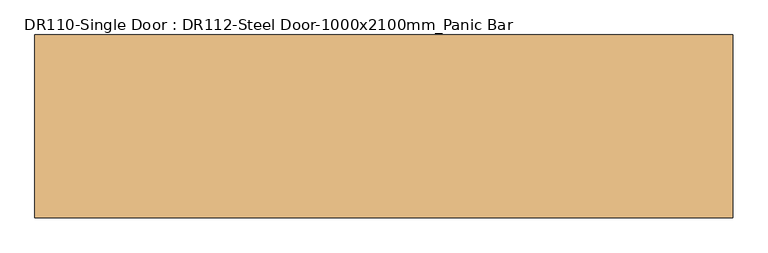
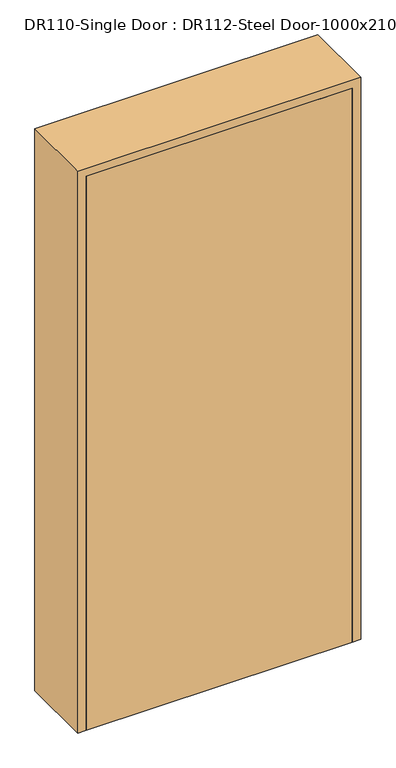
"""IFC4 building model written with IfcOpenShell, lengths in millimetres: door geometry, DR110-Single Door : DR112-Steel Door-1000x2100mm_Panic Bar."""

from ifc_helpers import new_model, si_unit, origin, origin_with_axes, place, context, project, spatial, polyline, outline, extrude, faceted_brep, source, transform, mapped, element, save


def dr110_single_door_dr112_steel_door_1000x2100mm_panic_bar_81a01685(model_context):
    return source(origin(), model_context, "Body", "SolidModel", [
        extrude(outline(polyline([(470.0, -131.0), (-470.0, -131.0), (-470.0, -96.0), (470.0, -96.0), (470.0, -131.0)])), origin_with_axes(), (0.0, 0.0, 1.0), 2070.0),
        faceted_brep([(470.0, -131.0, 0.0), (470.0, -96.0, 0.0), (450.0, -96.0, 0.0), (450.0, 96.0, 0.0), (470.0, 96.0, 0.0), (470.0, 131.0, 0.0), (500.0, 131.0, 0.0), (500.0, -131.0, 0.0), (500.0, -131.0, 2100.0), (-500.0, -131.0, 2100.0), (-500.0, -131.0, 0.0), (-470.0, -131.0, 0.0), (-470.0, -131.0, 2070.0), (470.0, -131.0, 2070.0), (500.0, 131.0, 2100.0), (470.0, 131.0, 2070.0), (-470.0, 131.0, 2070.0), (-470.0, 131.0, 0.0), (-500.0, 131.0, 0.0), (-500.0, 131.0, 2100.0), (470.0, 96.0, 2070.0), (450.0, 96.0, 2050.0), (-450.0, 96.0, 2050.0), (-450.0, 96.0, 0.0), (-470.0, 96.0, 0.0), (-470.0, 96.0, 2070.0), (450.0, -96.0, 2050.0), (470.0, -96.0, 2070.0), (-470.0, -96.0, 2070.0), (-470.0, -96.0, 0.0), (-450.0, -96.0, 0.0), (-450.0, -96.0, 2050.0)], [[[0, 1, 2, 3, 4, 5, 6, 7]], [[7, 8, 9, 10, 11, 12, 13, 0]], [[6, 14, 8, 7]], [[5, 15, 16, 17, 18, 19, 14, 6]], [[4, 20, 15, 5]], [[3, 21, 22, 23, 24, 25, 20, 4]], [[2, 26, 21, 3]], [[1, 27, 28, 29, 30, 31, 26, 2]], [[0, 13, 27, 1]], [[12, 11, 29, 28]], [[11, 10, 18, 17, 24, 23, 30, 29]], [[19, 18, 10, 9]], [[25, 24, 17, 16]], [[31, 30, 23, 22]], [[14, 19, 9, 8]], [[20, 25, 16, 15]], [[26, 31, 22, 21]], [[13, 12, 28, 27]]]),
    ])


if __name__ == "__main__":
    model = new_model("IFC4")
    model_context = context("Model", 3, world=origin())
    ifc_project = project(units=[si_unit("LENGTHUNIT", "METRE", prefix="MILLI")], contexts=[model_context])
    site = spatial("IfcSite", under=ifc_project)
    building = spatial("IfcBuilding", under=site)
    placement = place(None, origin())
    dr110_single_door_dr112_steel_door_1000x2100mm_panic_bar_shape = dr110_single_door_dr112_steel_door_1000x2100mm_panic_bar_81a01685(model_context)
    element("IfcDoor", 1, ObjectType="DR110-Single Door : DR112-Steel Door-1000x2100mm_Panic Bar", at=placement, inside=building, context=model_context, shape_type="MappedRepresentation", body=[
        mapped(dr110_single_door_dr112_steel_door_1000x2100mm_panic_bar_shape, transform((0.0, 0.0, 0.0), x_axis=(1.0, 0.0, 0.0), y_axis=(0.0, 1.0, 0.0), z_axis=(0.0, 0.0, 1.0))),
    ])
    save(model, "model.ifc")

# Revit data of these elements
# Type "DR110-Single Door : DR112-Steel Door-1000x2100mm_Panic Bar"
#   Type Mark = "SD"
#   Analytic Construction = "<None>"
#   프레임 투영 외부. = 25 mm
#   프레임 투영 내부. = 25 mm
#   프레임 폭 = 75 mm
#   Height = 2100 mm
#   Width = 1000 mm
#   Define Thermal Properties by = 1
#   문 패널 = SD1 문 패널
#   문 프레임 = A04AQ098-00002_Steel Door_non FP_single
#   Function = (empty or 0)
#   Wall Closure = (empty or 0)
# Element 1 (IfcDoor, "DR110-Single Door : DR112-Steel Door-1000x2100mm_Panic Bar")
#   Materials on its faces: "A04AQ098-00002_Steel Door_non FP_single", "SD1 문 패널"
# Materials
#   "SD1 문 패널": class "금속", colour RGB 247 247 247, transparency 0, Description = "STEEL DOOR (1000Wx2100H)"
#   "A04AQ098-00002_Steel Door_non FP_single": class "금속", colour RGB 247 247 247, transparency 0, Description = "Steel Door", W00) Work Master Code = "A04AQ098-00002", W01) Work Master_Lv1 = "Finishing Work", W02) Work Master_Lv2 = "Door & Window Work", W03) Work Master_Spec.1 = "Steel Door w/ Steel Frame", W04) Work Master_Spec.2 = "Fire Protective Rating: N/A, Single Door", W05) Work Master_Spec.3 = "w/ Hardware & Accessories", Cost = 0
